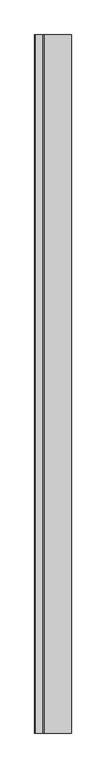
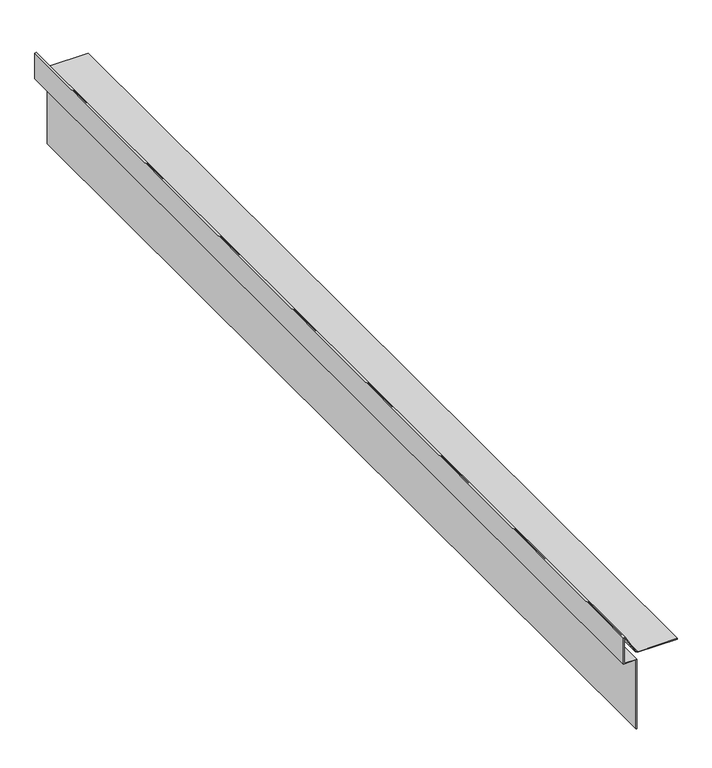
"""IFC4 building model written with IfcOpenShell, lengths in millimetres: proxy geometry, GRAVEL STOP16:GRAVEL STOP002:305426 : GRAVEL STOP16:GRAVEL STOP002:305426."""

from ifc_helpers import new_model, si_unit, frame, origin, place, context, project, spatial, polyline, outline, extrude, source, transform, mapped, element, save


def generic_models_1e7da119(model_context):
    return source(origin(), model_context, "Body", "SweptSolid", [
        extrude(outline(polyline([(40259.5408757, 1993.3009663), (40295.3431515, 1972.6305128), (40294.5307525, 1969.5985985), (40240.9633674, 1969.5985985), (40240.9633674, 1993.938336), (40097.9858473, 1993.938336), (40097.9858473, 1995.349447), (40242.3744784, 1995.349447), (40242.3744784, 1971.0097095), (40293.447969, 1971.0097095), (40293.699878, 1971.9498466), (40258.5078708, 1992.2679614), (40255.9633674, 1996.6751705), (40255.9633674, 2074.5111832), (40257.3744784, 2074.5111832), (40257.3744784, 1997.0532766), (40259.5408757, 1993.3009663)])), frame((0.0, 1278.3325412, 0.0), z_axis=(0.0, 1.0, 0.0), x_axis=(0.0, 0.0, 1.0)), (0.0, 0.0, 1.0), 2000.25),
    ])


if __name__ == "__main__":
    model = new_model("IFC4")
    model_context = context("Model", 3, world=origin())
    ifc_project = project(units=[si_unit("LENGTHUNIT", "METRE", prefix="MILLI")], contexts=[model_context])
    site = spatial("IfcSite", under=ifc_project)
    building = spatial("IfcBuilding", under=site)
    placement = place(None, origin())
    generic_models_shape = generic_models_1e7da119(model_context)
    element("IfcBuildingElementProxy", 1, Name="GRAVEL STOP16:GRAVEL STOP002:305426 : GRAVEL STOP16:GRAVEL STOP002:305426", ObjectType="GRAVEL STOP16:GRAVEL STOP002:305426 : GRAVEL STOP16:GRAVEL STOP002:305426", at=placement, inside=building, context=model_context, shape_type="MappedRepresentation", body=[
        mapped(generic_models_shape, transform((0.0, 0.0, 0.0), x_axis=(1.0, 0.0, 0.0), y_axis=(0.0, 1.0, 0.0), z_axis=(0.0, 0.0, 1.0))),
    ])
    save(model, "model.ifc")

# Revit data of these elements
# Type "GRAVEL STOP16:GRAVEL STOP002:305426 : GRAVEL STOP16:GRAVEL STOP002:305426"
#   NameOverride = "GRAVEL STOP16:GRAVEL STOP002:305426"
#   ObjectTypeOverride = "GRAVEL STOP16:GRAVEL STOP002"
#   Reference = "GRAVEL STOP002"
#   Category = "Generic Models"
#   Tag = "305426"
# Element 1 (IfcBuildingElementProxy, "GRAVEL STOP16:GRAVEL STOP002:305426 : GRAVEL STOP16:GRAVEL STOP002:305426")
#   Materials on its faces: "GRAVEL STOP REQUIRED WITH GRAVEL SURFACE SYSTEMS"
# Materials
#   "GRAVEL STOP REQUIRED WITH GRAVEL SURFACE SYSTEMS": class "Unassigned", colour RGB 170 170 127, transparency 0, Cost = 0
